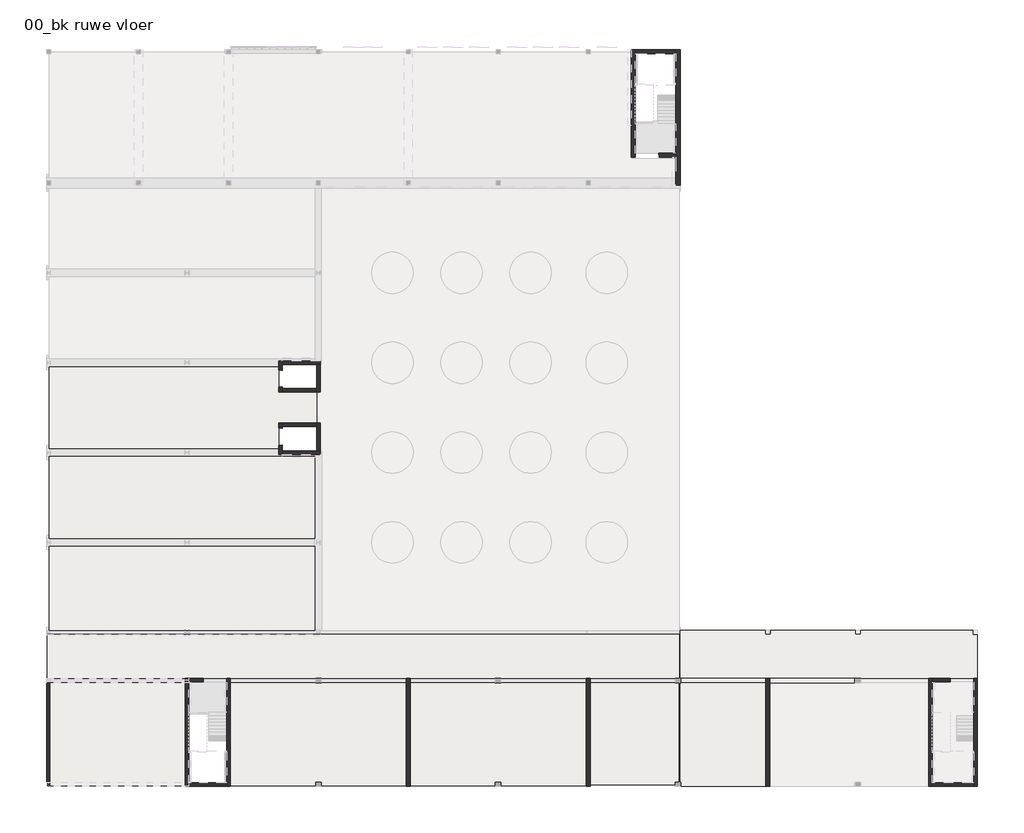
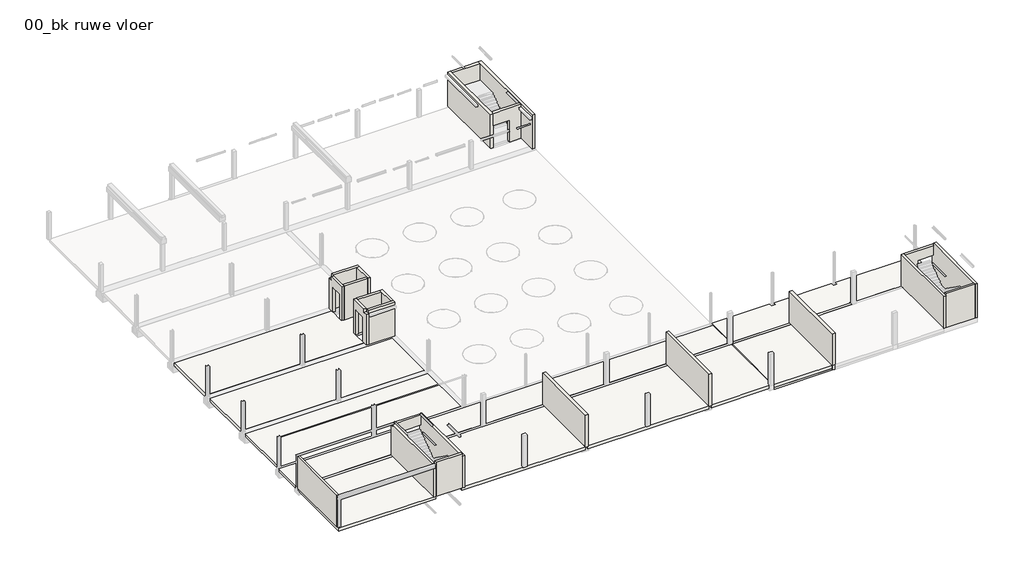
# One storey, part 1 of 6: 24 walls, 18 slabs.
"""IFC4 building model written with IfcOpenShell, lengths in millimetres."""

from ifc_helpers import new_model, si_unit, frame, origin, place, context, project, spatial, polyline, outline, extrude, faceted_brep, element, save

model = new_model("IFC4")

# Units and contexts
model_context = context("Model", 3, world=origin())
ifc_project = project(units=[si_unit("LENGTHUNIT", "METRE", prefix="MILLI")], contexts=[model_context])

# Site, building, storey
site = spatial("IfcSite", under=ifc_project)
building = spatial("IfcBuilding", under=site)
storey = spatial("IfcBuildingStorey", under=building, Name="00_bk ruwe vloer", Elevation=-70.0)

# Slabs
placement = place(None, origin())
element("IfcSlab", 1, ObjectType="NLRS_23_FL_isolatieplaatvloer 320_gen_rsf", at=placement, inside=storey, context=model_context, shape_type="Brep", body=[
    faceted_brep([(52150.0, 7650.0, -390.0), (52150.0, 11150.0, -390.0), (58300.0, 11150.0, -390.0), (58300.0, 10850.0, -390.0), (58700.0, 10850.0, -390.0), (58700.0, 11150.0, -390.0), (64800.0, 11150.0, -390.0), (64800.0, 10850.0, -390.0), (65200.0, 10850.0, -390.0), (65200.0, 11150.0, -390.0), (73300.0, 11150.0, -390.0), (73300.0, 10800.0, -390.0), (73650.0, 10800.0, -390.0), (73650.0, 7650.0, -390.0), (65250.0, 7650.0, -390.0), (65250.0, 7700.0, -390.0), (64750.0, 7700.0, -390.0), (64750.0, 7650.0, -390.0), (52150.0, 7650.0, -70.0), (64750.0, 7650.0, -70.0), (64750.0, 7700.0, -70.0), (65250.0, 7700.0, -70.0), (65250.0, 7650.0, -70.0), (73650.0, 7650.0, -70.0), (73650.0, 10800.0, -70.0), (73300.0, 10800.0, -70.0), (73300.0, 11150.0, -70.0), (65200.0, 11150.0, -70.0), (65200.0, 10850.0, -70.0), (64800.0, 10850.0, -70.0), (64800.0, 11150.0, -70.0), (58700.0, 11150.0, -70.0), (58700.0, 10850.0, -70.0), (58300.0, 10850.0, -70.0), (58300.0, 11150.0, -70.0), (52150.0, 11150.0, -70.0), (52150.0, 10850.0, -70.0)], [[[0, 1, 2, 3, 4, 5, 6, 7, 8, 9, 10, 11, 12, 13, 14, 15, 16, 17]], [[18, 19, 20, 21, 22, 23, 24, 25, 26, 27, 28, 29, 30, 31, 32, 33, 34, 35, 36]], [[1, 0, 18, 36, 35]], [[10, 9, 27, 26]], [[13, 12, 24, 23]], [[0, 17, 19, 18]], [[14, 13, 23, 22]], [[15, 14, 22, 21]], [[16, 15, 21, 20]], [[17, 16, 20, 19]], [[2, 1, 35, 34]], [[3, 2, 34, 33]], [[4, 3, 33, 32]], [[5, 4, 32, 31]], [[6, 5, 31, 30]], [[7, 6, 30, 29]], [[8, 7, 29, 28]], [[9, 8, 28, 27]], [[11, 10, 26, 25]], [[12, 11, 25, 24]]]),
])
element("IfcSlab", 2, ObjectType="NLRS_23_FL_breedplaat 320_gen_rsf", at=placement, inside=storey, context=model_context, shape_type="Brep", body=[
    faceted_brep([(6410.0, 7350.0, -390.0), (16375.0, 7350.0, -390.0), (16625.0, 7350.0, -390.0), (16625.0, 150.0, -390.0), (16625.0, -90.0, -390.0), (6650.0, -90.0, -390.0), (6410.0, -90.0, -390.0), (6410.0, 7150.0, -390.0), (16400.0, 125.0, -390.0), (16400.0, 7175.0, -390.0), (6625.0, 7175.0, -390.0), (6625.0, 125.0, -390.0), (16625.0, 7350.0, -70.0), (6410.0, 7350.0, -70.0), (6410.0, -90.0, -70.0), (6650.0, -90.0, -70.0), (16625.0, -90.0, -70.0), (16625.0, 150.0, -70.0), (6625.0, 7175.0, -330.0), (16400.0, 7175.0, -330.0), (16400.0, 125.0, -330.0), (6625.0, 125.0, -330.0)], [[[0, 1, 2, 3, 4, 5, 6, 7], [8, 9, 10, 11]], [[12, 13, 14, 15, 16, 17]], [[2, 1, 0, 13, 12]], [[4, 3, 2, 12, 17, 16]], [[6, 5, 4, 16, 15, 14]], [[0, 7, 6, 14, 13]], [[18, 19, 20, 21]], [[20, 19, 9, 8]], [[21, 20, 8, 11]], [[18, 21, 11, 10]], [[19, 18, 10, 9]]]),
])
element("IfcSlab", 3, ObjectType="NLRS_23_FL_breedplaat 320_gen_rsf", at=placement, inside=storey, context=model_context, shape_type="Brep", body=[
    faceted_brep([(52090.0, 10850.0, -390.0), (52090.0, 10650.0, -390.0), (52090.0, 7850.0, -390.0), (52090.0, 7650.0, -390.0), (19375.0, 7650.0, -390.0), (16625.0, 7650.0, -390.0), (16375.0, 7650.0, -390.0), (6410.0, 7650.0, -390.0), (6410.0, 7850.0, -390.0), (6410.0, 10650.0, -390.0), (6410.0, 10850.0, -390.0), (51875.0, 7825.0, -390.0), (51875.0, 10675.0, -390.0), (6625.0, 10675.0, -390.0), (6625.0, 7825.0, -390.0), (52090.0, 7650.0, -70.0), (52090.0, 10850.0, -70.0), (6410.0, 10850.0, -70.0), (6410.0, 7650.0, -70.0), (16625.0, 7650.0, -70.0), (19375.0, 7650.0, -70.0), (6625.0, 10675.0, -330.0), (51875.0, 10675.0, -330.0), (51875.0, 7825.0, -330.0), (6625.0, 7825.0, -330.0)], [[[0, 1, 2, 3, 4, 5, 6, 7, 8, 9, 10], [11, 12, 13, 14]], [[15, 16, 17, 18, 19, 20]], [[3, 2, 1, 0, 16, 15]], [[7, 6, 5, 4, 3, 15, 20, 19, 18]], [[10, 9, 8, 7, 18, 17]], [[0, 10, 17, 16]], [[21, 22, 23, 24]], [[23, 22, 12, 11]], [[24, 23, 11, 14]], [[21, 24, 14, 13]], [[22, 21, 13, 12]]]),
])
element("IfcSlab", 4, ObjectType="NLRS_23_FL_isolatieplaatvloer 320_gen_rsf", at=placement, inside=storey, context=model_context, shape_type="Brep", body=[
    faceted_brep([(25750.0, 17200.0, -390.0), (25750.0, 11350.0, -390.0), (25750.0, 11150.0, -390.0), (6550.0, 11150.0, -390.0), (6550.0, 11350.0, -390.0), (6550.0, 17000.0, -390.0), (6550.0, 17200.0, -390.0), (25500.0, 17200.0, -390.0), (25550.0, 17200.0, -390.0), (25700.0, 17200.0, -390.0), (25750.0, 17200.0, -70.0), (25700.0, 17200.0, -70.0), (6550.0, 17200.0, -70.0), (6550.0, 11150.0, -70.0), (25750.0, 11150.0, -70.0)], [[[0, 1, 2, 3, 4, 5, 6, 7, 8, 9]], [[10, 11, 12, 13, 14]], [[2, 1, 0, 10, 14]], [[3, 2, 14, 13]], [[6, 5, 4, 3, 13, 12]], [[0, 9, 8, 7, 6, 12, 11, 10]]]),
])
element("IfcSlab", 5, ObjectType="NLRS_23_FL_isolatieplaatvloer 320_gen_rsf", at=placement, inside=storey, context=model_context, shape_type="Brep", body=[
    faceted_brep([(25750.0, 23700.0, -390.0), (25750.0, 17800.0, -390.0), (25700.0, 17800.0, -390.0), (25550.0, 17800.0, -390.0), (25500.0, 17800.0, -390.0), (6550.0, 17800.0, -390.0), (6550.0, 18000.0, -390.0), (6550.0, 23500.0, -390.0), (6550.0, 23700.0, -390.0), (25500.0, 23700.0, -390.0), (25550.0, 23700.0, -390.0), (25700.0, 23700.0, -390.0), (25750.0, 23700.0, -70.0), (25700.0, 23700.0, -70.0), (6550.0, 23700.0, -70.0), (6550.0, 17800.0, -70.0), (25700.0, 17800.0, -70.0), (25750.0, 17800.0, -70.0)], [[[0, 1, 2, 3, 4, 5, 6, 7, 8, 9, 10, 11]], [[12, 13, 14, 15, 16, 17]], [[1, 0, 12, 17]], [[5, 4, 3, 2, 1, 17, 16, 15]], [[8, 7, 6, 5, 15, 14]], [[0, 11, 10, 9, 8, 14, 13, 12]]]),
])
element("IfcSlab", 6, ObjectType="NLRS_23_FL_isolatieplaatvloer 320_gen_rsf", at=placement, inside=storey, context=model_context, shape_type="Brep", body=[
    faceted_brep([(23125.0, 30200.0, -390.0), (23125.0, 30000.0, -390.0), (23125.0, 28475.0, -390.0), (23375.0, 28475.0, -390.0), (25875.0, 28475.0, -390.0), (25875.0, 28375.0, -390.0), (25875.0, 26125.0, -390.0), (25875.0, 26025.0, -390.0), (23375.0, 26025.0, -390.0), (23125.0, 26025.0, -390.0), (23125.0, 24500.0, -390.0), (23125.0, 24300.0, -390.0), (6550.0, 24300.0, -390.0), (6550.0, 24500.0, -390.0), (6550.0, 30000.0, -390.0), (6550.0, 30200.0, -390.0), (23125.0, 30200.0, -70.0), (6550.0, 30200.0, -70.0), (6550.0, 24300.0, -70.0), (23125.0, 24300.0, -70.0), (23125.0, 26025.0, -70.0), (23375.0, 26025.0, -70.0), (25875.0, 26025.0, -70.0), (25875.0, 28475.0, -70.0), (23375.0, 28475.0, -70.0), (23125.0, 28475.0, -70.0)], [[[0, 1, 2, 3, 4, 5, 6, 7, 8, 9, 10, 11, 12, 13, 14, 15]], [[16, 17, 18, 19, 20, 21, 22, 23, 24, 25]], [[2, 1, 0, 16, 25]], [[12, 11, 19, 18]], [[15, 14, 13, 12, 18, 17]], [[0, 15, 17, 16]], [[4, 3, 2, 25, 24, 23]], [[7, 6, 5, 4, 23, 22]], [[9, 8, 7, 22, 21, 20]], [[11, 10, 9, 20, 19]]]),
])
element("IfcSlab", 7, ObjectType="NLRS_23_FL_breedplaat 320_gen_rsf", at=placement, inside=storey, context=model_context, shape_type="Brep", body=[
    faceted_brep([(32350.0, 7350.0, -390.0), (32350.0, 150.0, -390.0), (32350.0, -90.0, -390.0), (19375.0, -90.0, -390.0), (19375.0, 150.0, -390.0), (19375.0, 7350.0, -390.0), (32175.0, 125.0, -390.0), (32175.0, 7175.0, -390.0), (19600.0, 7175.0, -390.0), (19600.0, 125.0, -390.0), (32350.0, -90.0, -70.0), (32350.0, 150.0, -70.0), (32350.0, 7350.0, -70.0), (19375.0, 7350.0, -70.0), (19375.0, 150.0, -70.0), (19375.0, -90.0, -70.0), (19600.0, 7175.0, -330.0), (32175.0, 7175.0, -330.0), (32175.0, 125.0, -330.0), (19600.0, 125.0, -330.0)], [[[0, 1, 2, 3, 4, 5], [6, 7, 8, 9]], [[10, 11, 12, 13, 14, 15]], [[2, 1, 0, 12, 11, 10]], [[3, 2, 10, 15]], [[5, 4, 3, 15, 14, 13]], [[0, 5, 13, 12]], [[16, 17, 18, 19]], [[18, 17, 7, 6]], [[19, 18, 6, 9]], [[16, 19, 9, 8]], [[17, 16, 8, 7]]]),
])
element("IfcSlab", 8, ObjectType="NLRS_23_FL_breedplaat 320_gen_rsf", at=placement, inside=storey, context=model_context, shape_type="Brep", body=[
    faceted_brep([(45350.0, 7350.0, -390.0), (45350.0, 7150.0, -390.0), (45350.0, 150.0, -390.0), (45350.0, -90.0, -390.0), (32650.0, -90.0, -390.0), (32650.0, 150.0, -390.0), (32650.0, 7150.0, -390.0), (32650.0, 7350.0, -390.0), (45175.0, 125.0, -390.0), (45175.0, 7175.0, -390.0), (32825.0, 7175.0, -390.0), (32825.0, 125.0, -390.0), (45350.0, -90.0, -70.0), (45350.0, 150.0, -70.0), (45350.0, 7350.0, -70.0), (32650.0, 7350.0, -70.0), (32650.0, 150.0, -70.0), (32650.0, -90.0, -70.0), (32825.0, 7175.0, -330.0), (45175.0, 7175.0, -330.0), (45175.0, 125.0, -330.0), (32825.0, 125.0, -330.0)], [[[0, 1, 2, 3, 4, 5, 6, 7], [8, 9, 10, 11]], [[12, 13, 14, 15, 16, 17]], [[3, 2, 1, 0, 14, 13, 12]], [[4, 3, 12, 17]], [[7, 6, 5, 4, 17, 16, 15]], [[0, 7, 15, 14]], [[18, 19, 20, 21]], [[20, 19, 9, 8]], [[21, 20, 8, 11]], [[18, 21, 11, 10]], [[19, 18, 10, 9]]]),
])
element("IfcSlab", 9, ObjectType="NLRS_23_FL_breedplaat 320_gen_rsf", at=placement, inside=storey, context=model_context, shape_type="Brep", body=[
    faceted_brep([(52050.0, 7350.0, -390.0), (52050.0, 7150.0, -390.0), (52050.0, 150.0, -390.0), (52050.0, -50.0, -390.0), (51750.0, -50.0, -390.0), (45650.0, -50.0, -390.0), (45650.0, 150.0, -390.0), (45650.0, 7150.0, -390.0), (45650.0, 7350.0, -390.0), (51875.0, 125.0, -390.0), (51875.0, 7175.0, -390.0), (45825.0, 7175.0, -390.0), (45825.0, 125.0, -390.0), (52050.0, -50.0, -70.0), (52050.0, 150.0, -70.0), (52050.0, 7350.0, -70.0), (45650.0, 7350.0, -70.0), (45650.0, 150.0, -70.0), (45650.0, -50.0, -70.0), (51750.0, -50.0, -70.0), (45825.0, 7175.0, -330.0), (51875.0, 7175.0, -330.0), (51875.0, 125.0, -330.0), (45825.0, 125.0, -330.0)], [[[0, 1, 2, 3, 4, 5, 6, 7, 8], [9, 10, 11, 12]], [[13, 14, 15, 16, 17, 18, 19]], [[3, 2, 1, 0, 15, 14, 13]], [[5, 4, 3, 13, 19, 18]], [[8, 7, 6, 5, 18, 17, 16]], [[0, 8, 16, 15]], [[20, 21, 22, 23]], [[22, 21, 10, 9]], [[23, 22, 9, 12]], [[20, 23, 12, 11]], [[21, 20, 11, 10]]]),
])
element("IfcSlab", 10, ObjectType="NLRS_23_FL_isolatieplaatvloer 320_gen_rsf", at=placement, inside=storey, context=model_context, shape_type="SweptSolid", body=[
    extrude(outline(polyline([(58350.0, 7350.0), (58350.0, -150.0), (52250.0, -150.0), (52250.0, 150.0), (52150.0, 150.0), (52150.0, 7350.0), (58350.0, 7350.0)])), frame((0.0, 0.0, -390.0), z_axis=(0.0, 0.0, 1.0), x_axis=(1.0, 0.0, 0.0)), (0.0, 0.0, 1.0), 320.0),
])
element("IfcSlab", 11, ObjectType="NLRS_23_FL_beton ihwg vloeraanstort 520_gen_rsf", at=placement, inside=storey, context=model_context, shape_type="Brep", body=[
    faceted_brep([(64750.0, 7650.0, -590.0), (64750.0, 7350.0, -590.0), (58650.0, 7350.0, -590.0), (58650.0, -150.0, -590.0), (58350.0, -150.0, -590.0), (58350.0, 7350.0, -590.0), (52150.0, 7350.0, -590.0), (52150.0, 7650.0, -590.0), (64750.0, 7650.0, -70.0), (52200.0, 7650.0, -70.0), (52150.0, 7650.0, -70.0), (52150.0, 7350.0, -70.0), (52200.0, 7350.0, -70.0), (58350.0, 7350.0, -70.0), (58350.0, -150.0, -70.0), (58650.0, -150.0, -70.0), (58650.0, 7350.0, -70.0), (64750.0, 7350.0, -70.0), (52150.0, 7350.0, -390.0), (52150.0, 7650.0, -390.0)], [[[0, 1, 2, 3, 4, 5, 6, 7]], [[8, 9, 10, 11, 12, 13, 14, 15, 16, 17]], [[1, 0, 8, 17]], [[2, 1, 17, 16]], [[3, 2, 16, 15]], [[4, 3, 15, 14]], [[5, 4, 14, 13]], [[6, 5, 13, 12, 11, 18]], [[7, 6, 18, 11, 10, 19]], [[0, 7, 19, 10, 9, 8]]]),
])
element("IfcSlab", 12, ObjectType="NLRS_23_FL_isolatie isolatieplaatvloer 200_gen_rsf", at=placement, inside=storey, context=model_context, shape_type="Brep", body=[
    faceted_brep([(52150.0, 7650.0, -590.0), (52150.0, 7800.0, -590.0), (52150.0, 10750.0, -590.0), (52150.0, 11150.0, -590.0), (58300.0, 11150.0, -590.0), (58300.0, 10850.0, -590.0), (58700.0, 10850.0, -590.0), (58700.0, 11150.0, -590.0), (64800.0, 11150.0, -590.0), (64800.0, 10850.0, -590.0), (65200.0, 10850.0, -590.0), (65200.0, 11150.0, -590.0), (73300.0, 11150.0, -590.0), (73300.0, 10800.0, -590.0), (73650.0, 10800.0, -590.0), (73650.0, 7650.0, -590.0), (65250.0, 7650.0, -590.0), (65250.0, 7700.0, -590.0), (64750.0, 7700.0, -590.0), (64750.0, 7650.0, -590.0), (52150.0, 7650.0, -390.0), (64750.0, 7650.0, -390.0), (64750.0, 7700.0, -390.0), (65250.0, 7700.0, -390.0), (65250.0, 7650.0, -390.0), (73650.0, 7650.0, -390.0), (73650.0, 10800.0, -390.0), (73300.0, 10800.0, -390.0), (73300.0, 11150.0, -390.0), (65200.0, 11150.0, -390.0), (65200.0, 10850.0, -390.0), (64800.0, 10850.0, -390.0), (64800.0, 11150.0, -390.0), (58700.0, 11150.0, -390.0), (58700.0, 10850.0, -390.0), (58300.0, 10850.0, -390.0), (58300.0, 11150.0, -390.0), (52150.0, 11150.0, -390.0), (52150.0, 10850.0, -390.0), (52150.0, 10650.0, -390.0), (52150.0, 7850.0, -390.0)], [[[0, 1, 2, 3, 4, 5, 6, 7, 8, 9, 10, 11, 12, 13, 14, 15, 16, 17, 18, 19]], [[20, 21, 22, 23, 24, 25, 26, 27, 28, 29, 30, 31, 32, 33, 34, 35, 36, 37, 38, 39, 40]], [[3, 2, 1, 0, 20, 40, 39, 38, 37]], [[12, 11, 29, 28]], [[15, 14, 26, 25]], [[0, 19, 21, 20]], [[16, 15, 25, 24]], [[17, 16, 24, 23]], [[18, 17, 23, 22]], [[19, 18, 22, 21]], [[4, 3, 37, 36]], [[5, 4, 36, 35]], [[6, 5, 35, 34]], [[7, 6, 34, 33]], [[8, 7, 33, 32]], [[9, 8, 32, 31]], [[10, 9, 31, 30]], [[11, 10, 30, 29]], [[13, 12, 28, 27]], [[14, 13, 27, 26]]]),
])
element("IfcSlab", 13, ObjectType="NLRS_23_FL_isolatie isolatieplaatvloer 200_gen_rsf", at=placement, inside=storey, context=model_context, shape_type="Brep", body=[
    faceted_brep([(58350.0, 7350.0, -590.0), (58350.0, -150.0, -590.0), (52250.0, -150.0, -590.0), (52250.0, 150.0, -590.0), (52150.0, 150.0, -590.0), (52150.0, 250.0, -590.0), (52150.0, 7200.0, -590.0), (52150.0, 7350.0, -590.0), (58350.0, 7350.0, -390.0), (52150.0, 7350.0, -390.0), (52150.0, 7150.0, -390.0), (52150.0, 150.0, -390.0), (52250.0, 150.0, -390.0), (52250.0, -150.0, -390.0), (58350.0, -150.0, -390.0)], [[[0, 1, 2, 3, 4, 5, 6, 7]], [[8, 9, 10, 11, 12, 13, 14]], [[1, 0, 8, 14]], [[2, 1, 14, 13]], [[7, 6, 5, 4, 11, 10, 9]], [[0, 7, 9, 8]], [[3, 2, 13, 12]], [[4, 3, 12, 11]]]),
])
element("IfcSlab", 14, ObjectType="NLRS_23_FL_breedplaat schil 60_gen_rsf", at=placement, inside=storey, context=model_context, shape_type="SweptSolid", body=[
    extrude(outline(polyline([(16400.0, 7175.0), (16400.0, 125.0), (6625.0, 125.0), (6625.0, 7175.0), (16400.0, 7175.0)])), frame((0.0, 0.0, -390.0), z_axis=(0.0, 0.0, 1.0), x_axis=(1.0, 0.0, 0.0)), (0.0, 0.0, 1.0), 60.0),
])
element("IfcSlab", 15, ObjectType="NLRS_23_FL_breedplaat schil 60_gen_rsf", at=placement, inside=storey, context=model_context, shape_type="SweptSolid", body=[
    extrude(outline(polyline([(32175.0, 7175.0), (32175.0, 125.0), (19600.0, 125.0), (19600.0, 7175.0), (32175.0, 7175.0)])), frame((0.0, 0.0, -390.0), z_axis=(0.0, 0.0, 1.0), x_axis=(1.0, 0.0, 0.0)), (0.0, 0.0, 1.0), 60.0),
])
element("IfcSlab", 16, ObjectType="NLRS_23_FL_breedplaat schil 60_gen_rsf", at=placement, inside=storey, context=model_context, shape_type="SweptSolid", body=[
    extrude(outline(polyline([(45175.0, 7175.0), (45175.0, 125.0), (32825.0, 125.0), (32825.0, 7175.0), (45175.0, 7175.0)])), frame((0.0, 0.0, -390.0), z_axis=(0.0, 0.0, 1.0), x_axis=(1.0, 0.0, 0.0)), (0.0, 0.0, 1.0), 60.0),
])
element("IfcSlab", 17, ObjectType="NLRS_23_FL_breedplaat schil 60_gen_rsf", at=placement, inside=storey, context=model_context, shape_type="SweptSolid", body=[
    extrude(outline(polyline([(51875.0, 7175.0), (51875.0, 125.0), (45825.0, 125.0), (45825.0, 7175.0), (51875.0, 7175.0)])), frame((0.0, 0.0, -390.0), z_axis=(0.0, 0.0, 1.0), x_axis=(1.0, 0.0, 0.0)), (0.0, 0.0, 1.0), 60.0),
])
element("IfcSlab", 18, ObjectType="NLRS_23_FL_breedplaat schil 60_gen_rsf", at=placement, inside=storey, context=model_context, shape_type="SweptSolid", body=[
    extrude(outline(polyline([(51875.0, 10675.0), (51875.0, 7825.0), (6625.0, 7825.0), (6625.0, 10675.0), (51875.0, 10675.0)])), frame((0.0, 0.0, -390.0), z_axis=(0.0, 0.0, 1.0), x_axis=(1.0, 0.0, 0.0)), (0.0, 0.0, 1.0), 60.0),
])

# Walls
element("IfcWall", 19, ObjectType="NLRS_22_WA_beton ihw 250_gen_rsf", at=placement, inside=storey, context=model_context, shape_type="Brep", body=[
    faceted_brep([(19625.0, -150.0, -70.0), (19625.0, 7650.0, -70.0), (19625.0, 7650.0, 3470.0), (19625.0, -150.0, 3470.0), (19375.0, -150.0, -70.0), (19375.0, -150.0, 3470.0), (19375.0, 7400.0, 3470.0), (19375.0, 7650.0, 3470.0), (19375.0, 7650.0, 2370.0), (19375.0, 7650.0, -70.0), (19375.0, 7350.0, -70.0), (19375.0, 100.0, -70.0), (19375.0, -90.0, -70.0)], [[[0, 1, 2, 3]], [[4, 5, 6, 7, 8, 9, 10, 11, 12]], [[1, 0, 4, 12, 11, 10, 9]], [[2, 1, 9, 8, 7]], [[3, 2, 7, 6, 5]], [[0, 3, 5, 4]]]),
])
element("IfcWall", 20, ObjectType="NLRS_22_WA_beton ihw 250_gen_rsf", at=placement, inside=storey, context=model_context, shape_type="Brep", body=[
    faceted_brep([(16625.0, -150.0, -70.0), (16625.0, -90.0, -70.0), (16625.0, 100.0, -70.0), (16625.0, 7350.0, -70.0), (16625.0, 7400.0, -70.0), (16625.0, 7650.0, -70.0), (16625.0, 7650.0, 3320.0), (16625.0, 7330.0, 3320.0), (16625.0, 7330.0, 3470.0), (16625.0, 170.0, 3470.0), (16625.0, 170.0, 3090.0), (16625.0, -150.0, 3090.0), (16375.0, -150.0, -70.0), (16375.0, -150.0, 3090.0), (16375.0, 170.0, 3090.0), (16375.0, 170.0, 3470.0), (16375.0, 7330.0, 3470.0), (16375.0, 7330.0, 3320.0), (16375.0, 7650.0, 3320.0), (16375.0, 7650.0, -70.0)], [[[0, 1, 2, 3, 4, 5, 6, 7, 8, 9, 10, 11]], [[12, 13, 14, 15, 16, 17, 18, 19]], [[5, 4, 3, 2, 1, 0, 12, 19]], [[6, 5, 19, 18]], [[9, 8, 16, 15]], [[0, 11, 13, 12]], [[10, 9, 15, 14]], [[11, 10, 14, 13]], [[7, 6, 18, 17]], [[8, 7, 17, 16]]]),
])
element("IfcWall", 21, ObjectType="NLRS_22_WA_kalkzandsteen CS20 300_gen_rsf", at=placement, inside=storey, context=model_context, shape_type="SweptSolid", body=[
    extrude(outline(polyline([(32650.0, 7650.0), (32650.0, -150.0), (32350.0, -150.0), (32350.0, 7650.0), (32650.0, 7650.0)])), frame((0.0, 0.0, -70.0), z_axis=(0.0, 0.0, 1.0), x_axis=(1.0, 0.0, 0.0)), (0.0, 0.0, 1.0), 3540.0),
])
element("IfcWall", 22, ObjectType="NLRS_22_WA_kalkzandsteen CS20 300_gen_rsf", at=placement, inside=storey, context=model_context, shape_type="SweptSolid", body=[
    extrude(outline(polyline([(45650.0, 7650.0), (45650.0, -150.0), (45350.0, -150.0), (45350.0, 7650.0), (45650.0, 7650.0)])), frame((0.0, 0.0, -70.0), z_axis=(0.0, 0.0, 1.0), x_axis=(1.0, 0.0, 0.0)), (0.0, 0.0, 1.0), 3540.0),
])
element("IfcWall", 23, ObjectType="NLRS_22_WA_kalkzandsteen CS20 300_gen_rsf", at=placement, inside=storey, context=model_context, shape_type="SweptSolid", body=[
    extrude(outline(polyline([(58650.0, 7650.0), (58650.0, -150.0), (58350.0, -150.0), (58350.0, 7650.0), (58650.0, 7650.0)])), frame((0.0, 0.0, -70.0), z_axis=(0.0, 0.0, 1.0), x_axis=(1.0, 0.0, 0.0)), (0.0, 0.0, 1.0), 3540.0),
])
element("IfcWall", 24, ObjectType="NLRS_21_WA_beton ihw 250_gen_rsf", at=placement, inside=storey, context=model_context, shape_type="Brep", body=[
    faceted_brep([(73650.0, -150.0, -70.0), (73650.0, 7650.0, -70.0), (73650.0, 7650.0, 3470.0), (73650.0, 7400.0, 3470.0), (73650.0, 7400.0, 3730.0), (73650.0, -150.0, 3730.0), (73400.0, -150.0, -70.0), (73400.0, -150.0, 3730.0), (73400.0, 100.0, 3730.0), (73400.0, 7400.0, 3730.0), (73400.0, 7400.0, 3470.0), (73400.0, 7650.0, 3470.0), (73400.0, 7650.0, 2370.0), (73400.0, 7650.0, -70.0), (73400.0, 7400.0, -70.0), (73400.0, 100.0, -70.0)], [[[0, 1, 2, 3, 4, 5]], [[6, 7, 8, 9, 10, 11, 12, 13, 14, 15]], [[1, 0, 6, 15, 14, 13]], [[2, 1, 13, 12, 11]], [[5, 4, 9, 8, 7]], [[0, 5, 7, 6]], [[3, 2, 11, 10]], [[4, 3, 10, 9]]]),
])
element("IfcWall", 25, ObjectType="NLRS_21_WA_kalkzandsteen CS12 214_gen_rsf", at=placement, inside=storey, context=model_context, shape_type="SweptSolid", body=[
    extrude(outline(polyline([(6564.0, 7330.0), (6564.0, 170.0), (6350.0, 170.0), (6350.0, 7330.0), (6564.0, 7330.0)])), frame((0.0, 0.0, -70.0), z_axis=(0.0, 0.0, 1.0), x_axis=(1.0, 0.0, 0.0)), (0.0, 0.0, 1.0), 3540.0),
])
element("IfcWall", 26, ObjectType="NLRS_21_WA_beton ihw 250_gen_rsf", at=placement, inside=storey, context=model_context, shape_type="Brep", body=[
    faceted_brep([(16625.0, -150.0, -70.0), (19375.0, -150.0, -70.0), (19375.0, -150.0, 3470.0), (19375.0, -150.0, 3730.0), (16625.0, -150.0, 3730.0), (16625.0, -150.0, 3470.0), (16625.0, -150.0, 3090.0), (19375.0, 100.0, -70.0), (16625.0, 100.0, -70.0), (16625.0, 100.0, 3730.0), (19375.0, 100.0, 3730.0), (19375.0, 100.0, 3470.0)], [[[0, 1, 2, 3, 4, 5, 6]], [[7, 8, 9, 10, 11]], [[1, 0, 8, 7]], [[1, 7, 11, 10, 3, 2]], [[4, 3, 10, 9]], [[0, 6, 5, 4, 9, 8]]]),
])
element("IfcWall", 27, ObjectType="NLRS_22_WA_beton ihw 250_gen_rsf", at=placement, inside=storey, context=model_context, shape_type="Brep", body=[
    faceted_brep([(19375.0, 7400.0, 3470.0), (16625.0, 7400.0, 3470.0), (16625.0, 7400.0, -70.0), (17675.0, 7400.0, -70.0), (17675.0, 7400.0, 2370.0), (19375.0, 7400.0, 2370.0), (16625.0, 7650.0, 3470.0), (19375.0, 7650.0, 3470.0), (19375.0, 7650.0, 2370.0), (17675.0, 7650.0, 2370.0), (17675.0, 7650.0, -70.0), (16625.0, 7650.0, -70.0), (16625.0, 7650.0, 3320.0)], [[[0, 1, 2, 3, 4, 5]], [[6, 7, 8, 9, 10, 11, 12]], [[2, 11, 10, 3]], [[7, 0, 5, 8]], [[1, 0, 7, 6]], [[2, 1, 6, 12, 11]], [[9, 4, 3, 10]], [[4, 9, 8, 5]]]),
])
element("IfcWall", 28, ObjectType="NLRS_22_WA_beton ihw 250_gen_rsf", at=placement, inside=storey, context=model_context, shape_type="Brep", body=[
    faceted_brep([(70375.0, -150.0, -70.0), (70375.0, 100.0, -70.0), (70375.0, 7400.0, -70.0), (70375.0, 7650.0, -70.0), (70375.0, 7650.0, 3470.0), (70375.0, 7400.0, 3470.0), (70375.0, -150.0, 3470.0), (70125.0, -150.0, -70.0), (70125.0, -150.0, 3470.0), (70125.0, 7650.0, 3470.0), (70125.0, 7650.0, -70.0), (70125.0, 7350.0, -70.0)], [[[0, 1, 2, 3, 4, 5, 6]], [[7, 8, 9, 10, 11]], [[3, 2, 1, 0, 7, 11, 10]], [[4, 3, 10, 9]], [[6, 5, 4, 9, 8]], [[0, 6, 8, 7]]]),
])
element("IfcWall", 29, ObjectType="NLRS_21_WA_beton ihw 250_gen_rsf", at=placement, inside=storey, context=model_context, shape_type="Brep", body=[
    faceted_brep([(70375.0, -150.0, -70.0), (73400.0, -150.0, -70.0), (73400.0, -150.0, 3730.0), (70375.0, -150.0, 3730.0), (70375.0, -150.0, 3470.0), (70375.0, 100.0, -70.0), (70375.0, 100.0, 3730.0), (73400.0, 100.0, 3730.0), (73400.0, 100.0, -70.0)], [[[0, 1, 2, 3, 4]], [[5, 6, 7, 8]], [[1, 0, 5, 8]], [[2, 1, 8, 7]], [[3, 2, 7, 6]], [[0, 4, 3, 6, 5]]]),
])
element("IfcWall", 30, ObjectType="NLRS_22_WA_beton ihw 250_gen_rsf", at=placement, inside=storey, context=model_context, shape_type="SweptSolid", body=[
    extrude(outline(polyline([(3470.0, 73400.0), (3470.0, 70375.0), (-70.0, 70375.0), (-70.0, 71700.0), (2370.0, 71700.0), (2370.0, 73400.0), (3470.0, 73400.0)])), frame((0.0, 7400.0, 0.0), z_axis=(0.0, 1.0, 0.0), x_axis=(0.0, 0.0, 1.0)), (0.0, 0.0, 1.0), 250.0),
])
element("IfcWall", 31, ObjectType="NLRS_22_WA_beton prefab 300_gen_rsf", at=placement, inside=storey, context=model_context, shape_type="Brep", body=[
    faceted_brep([(48905.0, 45350.0, -50.0), (48905.0, 53150.0, -50.0), (48905.0, 53150.0, 3730.0), (48905.0, 45350.0, 3730.0), (48605.0, 45350.0, -50.0), (48605.0, 45350.0, 3730.0), (48605.0, 53150.0, 3730.0), (48605.0, 53150.0, 3470.0), (48605.0, 53150.0, 3220.0), (48605.0, 53150.0, -50.0)], [[[0, 1, 2, 3]], [[4, 5, 6, 7, 8, 9]], [[1, 0, 4, 9]], [[2, 1, 9, 8, 7, 6]], [[3, 2, 6, 5]], [[0, 3, 5, 4]]]),
])
element("IfcWall", 32, ObjectType="NLRS_21_WA_beton prefab 300_gen_rsf", at=placement, inside=storey, context=model_context, shape_type="Brep", body=[
    faceted_brep([(52150.0, 43350.0, -50.0), (52150.0, 53150.0, -50.0), (52150.0, 53150.0, 3730.0), (52150.0, 43350.0, 3730.0), (51850.0, 43350.0, -50.0), (51850.0, 43350.0, 3220.0), (51850.0, 43350.0, 3470.0), (51850.0, 43350.0, 3730.0), (51850.0, 53150.0, 3730.0), (51850.0, 53150.0, -50.0)], [[[0, 1, 2, 3]], [[4, 5, 6, 7, 8, 9]], [[1, 0, 4, 9]], [[2, 1, 9, 8]], [[3, 2, 8, 7]], [[0, 3, 7, 6, 5, 4]]]),
])
element("IfcWall", 33, ObjectType="NLRS_21_WA_beton prefab 300_gen_rsf", at=placement, inside=storey, context=model_context, shape_type="SweptSolid", body=[
    extrude(outline(polyline([(48925.0, 53150.0), (51830.0, 53150.0), (51830.0, 52850.0), (48925.0, 52850.0), (48925.0, 53150.0)])), frame((0.0, 0.0, -50.0), z_axis=(0.0, 0.0, 1.0), x_axis=(1.0, 0.0, 0.0)), (0.0, 0.0, 1.0), 3780.0),
])
element("IfcWall", 34, ObjectType="NLRS_22_WA_beton prefab 300_gen_rsf", at=placement, inside=storey, context=model_context, shape_type="Brep", body=[
    faceted_brep([(48925.0, 45650.0, 3730.0), (51830.0, 45650.0, 3730.0), (51830.0, 45650.0, -50.0), (50625.0, 45650.0, -50.0), (50625.0, 45650.0, 2370.0), (48925.0, 45650.0, 2370.0), (51830.0, 45350.0, 3730.0), (48925.0, 45350.0, 3730.0), (48925.0, 45350.0, 2400.0), (50655.0, 45350.0, 2400.0), (50655.0, 45350.0, -50.0), (51830.0, 45350.0, -50.0)], [[[0, 1, 2, 3, 4, 5]], [[6, 7, 8, 9, 10, 11]], [[2, 11, 10, 3]], [[7, 0, 5, 8]], [[1, 0, 7, 6]], [[2, 1, 6, 11]], [[9, 4, 3, 10]], [[4, 9, 8, 5]]]),
])
element("IfcWall", 35, ObjectType="NLRS_22_WA_beton prefab 250_gen_rsf", at=placement, inside=storey, context=model_context, shape_type="Brep", body=[
    faceted_brep([(26125.0, 30625.0, -40.0), (23395.0, 30625.0, -40.0), (23395.0, 30625.0, 3150.0), (23395.0, 30625.0, 3400.0), (23395.0, 30625.0, 3730.0), (26125.0, 30625.0, 3730.0), (26125.0, 30625.0, 3400.0), (26125.0, 30625.0, 3150.0), (26125.0, 30375.0, -40.0), (26125.0, 30375.0, 3730.0), (23395.0, 30375.0, 3730.0), (23395.0, 30375.0, -40.0)], [[[0, 1, 2, 3, 4, 5, 6, 7]], [[8, 9, 10, 11]], [[1, 0, 8, 11]], [[4, 3, 2, 1, 11, 10]], [[5, 4, 10, 9]], [[0, 7, 6, 5, 9, 8]]]),
])
element("IfcWall", 36, ObjectType="NLRS_22_WA_beton prefab 250_gen_rsf", at=placement, inside=storey, context=model_context, shape_type="Brep", body=[
    faceted_brep([(23125.0, 28375.0, -40.0), (23125.0, 28375.0, 3730.0), (23125.0, 30231.5, 3730.0), (23125.0, 30231.5, 3355.0), (23125.0, 30625.0, 3355.0), (23125.0, 30625.0, -40.0), (23125.0, 29973.0, -40.0), (23125.0, 29973.0, 2705.0), (23125.0, 28723.0, 2705.0), (23125.0, 28723.0, -40.0), (23375.0, 28375.0, 3730.0), (23375.0, 28375.0, -40.0), (23375.0, 28748.0, -40.0), (23375.0, 28748.0, 2680.0), (23375.0, 29948.0, 2680.0), (23375.0, 29948.0, -40.0), (23375.0, 30625.0, -40.0), (23375.0, 30625.0, 3355.0), (23375.0, 30231.5, 3355.0), (23375.0, 30231.5, 3730.0)], [[[0, 1, 2, 3, 4, 5, 6, 7, 8, 9]], [[10, 11, 12, 13, 14, 15, 16, 17, 18, 19]], [[11, 0, 9, 12]], [[5, 16, 15, 6]], [[1, 0, 11, 10]], [[2, 1, 10, 19]], [[5, 4, 17, 16]], [[3, 2, 19, 18]], [[4, 3, 18, 17]], [[14, 7, 6, 15]], [[8, 13, 12, 9]], [[7, 14, 13, 8]]]),
])
element("IfcWall", 37, ObjectType="NLRS_22_WA_beton prefab 250_gen_rsf", at=placement, inside=storey, context=model_context, shape_type="SweptSolid", body=[
    extrude(outline(polyline([(25855.0, 28375.0), (23395.0, 28375.0), (23395.0, 28625.0), (25855.0, 28625.0), (25855.0, 28375.0)])), frame((0.0, 0.0, -40.0), z_axis=(0.0, 0.0, 1.0), x_axis=(1.0, 0.0, 0.0)), (0.0, 0.0, 1.0), 3770.0),
])
element("IfcWall", 38, ObjectType="NLRS_21_WA_beton prefab 250_gen_rsf", at=placement, inside=storey, context=model_context, shape_type="SweptSolid", body=[
    extrude(outline(polyline([(26125.0, 30355.0), (26125.0, 28375.0), (25875.0, 28375.0), (25875.0, 30355.0), (26125.0, 30355.0)])), frame((0.0, 0.0, -40.0), z_axis=(0.0, 0.0, 1.0), x_axis=(1.0, 0.0, 0.0)), (0.0, 0.0, 1.0), 3770.0),
])
element("IfcWall", 39, ObjectType="NLRS_22_WA_beton prefab 250_gen_rsf", at=placement, inside=storey, context=model_context, shape_type="SweptSolid", body=[
    extrude(outline(polyline([(23395.0, 26125.0), (25855.0, 26125.0), (25855.0, 25875.0), (23395.0, 25875.0), (23395.0, 26125.0)])), frame((0.0, 0.0, -40.0), z_axis=(0.0, 0.0, 1.0), x_axis=(1.0, 0.0, 0.0)), (0.0, 0.0, 1.0), 3770.0),
])
element("IfcWall", 40, ObjectType="NLRS_22_WA_beton prefab 250_gen_rsf", at=placement, inside=storey, context=model_context, shape_type="Brep", body=[
    faceted_brep([(23125.0, 23875.0, -40.0), (23125.0, 23875.0, 3355.0), (23125.0, 24291.5, 3355.0), (23125.0, 24291.5, 3730.0), (23125.0, 26125.0, 3730.0), (23125.0, 26125.0, -40.0), (23125.0, 25777.0, -40.0), (23125.0, 25777.0, 2705.0), (23125.0, 24527.0, 2705.0), (23125.0, 24527.0, -40.0), (23375.0, 23875.0, 3355.0), (23375.0, 23875.0, -40.0), (23375.0, 24552.0, -40.0), (23375.0, 24552.0, 2680.0), (23375.0, 25752.0, 2680.0), (23375.0, 25752.0, -40.0), (23375.0, 26125.0, -40.0), (23375.0, 26125.0, 3730.0), (23375.0, 24291.5, 3730.0), (23375.0, 24291.5, 3355.0)], [[[0, 1, 2, 3, 4, 5, 6, 7, 8, 9]], [[10, 11, 12, 13, 14, 15, 16, 17, 18, 19]], [[11, 0, 9, 12]], [[5, 16, 15, 6]], [[1, 0, 11, 10]], [[4, 3, 18, 17]], [[5, 4, 17, 16]], [[2, 1, 10, 19]], [[3, 2, 19, 18]], [[14, 7, 6, 15]], [[8, 13, 12, 9]], [[7, 14, 13, 8]]]),
])
element("IfcWall", 41, ObjectType="NLRS_22_WA_beton prefab 250_gen_rsf", at=placement, inside=storey, context=model_context, shape_type="Brep", body=[
    faceted_brep([(23395.0, 23875.0, -40.0), (26125.0, 23875.0, -40.0), (26125.0, 23875.0, 3150.0), (26125.0, 23875.0, 3400.0), (26125.0, 23875.0, 3730.0), (23395.0, 23875.0, 3730.0), (23395.0, 23875.0, 3400.0), (23395.0, 23875.0, 3150.0), (23395.0, 24125.0, -40.0), (23395.0, 24125.0, 3730.0), (26125.0, 24125.0, 3730.0), (26125.0, 24125.0, -40.0)], [[[0, 1, 2, 3, 4, 5, 6, 7]], [[8, 9, 10, 11]], [[1, 0, 8, 11]], [[4, 3, 2, 1, 11, 10]], [[5, 4, 10, 9]], [[0, 7, 6, 5, 9, 8]]]),
])
element("IfcWall", 42, ObjectType="NLRS_21_WA_beton prefab 250_gen_rsf", at=placement, inside=storey, context=model_context, shape_type="SweptSolid", body=[
    extrude(outline(polyline([(26125.0, 26125.0), (26125.0, 24145.0), (25875.0, 24145.0), (25875.0, 26125.0), (26125.0, 26125.0)])), frame((0.0, 0.0, -40.0), z_axis=(0.0, 0.0, 1.0), x_axis=(1.0, 0.0, 0.0)), (0.0, 0.0, 1.0), 3770.0),
])

save(model, "model.ifc")

# Revit data of these elements
# Type "NLRS_23_FL_isolatieplaatvloer 320_gen_rsf"
#   Keynote = ""
#   Type IfcGUID = "0X0KViByb4JPBOa4XaNeBK"
#   Type Comments = "d=320mm"
#   Description = "prefab isolatieplaatvloer, vrijdragend"
#   Assembly Code = "23.21"
#   IfcExportAs = "IfcSlab"
#   Function = 0
#   Layers, outside or top first: 40 mm "NLRS_f2_beton prefab_gen_rsf" (function 1); 235 mm "NLRS_f2_beton prefab_gen_rsf" (function 1); 45 mm "NLRS_f2_beton prefab_gen_rsf" (function 1)
# Type "NLRS_23_FL_breedplaat 320_gen_rsf"
#   Keynote = ""
#   Type IfcGUID = "1Sps1bgmr0zeLndh498PCM"
#   Type Comments = "d=320mm"
#   Description = "breedplaatvloer, vrijdragend"
#   Assembly Code = "23.21"
#   Type Mark = ""
#   IfcExportAs = "IfcSlab"
#   Function = 1
#   Layers, outside or top first: 320 mm "NLRS_f2_beton ihwg_gen_rsf" (function 1)
# Type "NLRS_23_FL_beton ihwg vloeraanstort 520_gen_rsf"
#   Keynote = ""
#   Type IfcGUID = "3aMdMHoe12P9KDGPyaIe$w"
#   Type Comments = "vloeraanstort d=520"
#   Description = "in het werk gestorte betonvloer, vrijdragend"
#   Assembly Code = "23.21"
#   IfcExportAs = "IfcSlab"
#   Function = 0
#   Layers, outside or top first: 520 mm "NLRS_f2_beton ihwg_gen_rsf" (function 1)
# Type "NLRS_23_FL_isolatie isolatieplaatvloer 200_gen_rsf"
#   Keynote = ""
#   Type IfcGUID = "3aMdMHoe12P9KDGPyaIfI8"
#   Type Comments = "d=200mm"
#   Description = "prefab isolatieplaatvloer, vrijdragend"
#   Assembly Code = "23.21"
#   IfcExportAs = "IfcSlab"
#   Function = 0
#   Layers, outside or top first: 200 mm "NLRS_n7_isolatie EPS_gen_rsf" (function 1)
# Type "NLRS_23_FL_breedplaat schil 60_gen_rsf"
#   Keynote = ""
#   Type IfcGUID = "3PAoVTCyX39AT9TmkNvccm"
#   Type Comments = "d=60mm"
#   Description = "prefab breedplaatvloer, vrijdragend"
#   Assembly Code = "23.21"
#   Type Mark = ""
#   IfcExportAs = "IfcSlab"
#   Function = 0
#   Layers, outside or top first: 60 mm "NLRS_f2_beton prefab_gen_rsf" (function 1)
# Type "NLRS_22_WA_beton ihw 250_gen_rsf"
#   Keynote = ""
#   Type IfcGUID = "1xcRxxwlX9cP9p3jVIop5v"
#   Description = "buitenwand beton ihw, generiek"
#   Assembly Code = "22.21"
#   IfcExportAs = "IfcWall"
#   Layers, outside or top first: 250 mm "NLRS_f2_beton ihwg_gen_rsf" (function 1)
# Type "NLRS_22_WA_kalkzandsteen CS20 300_gen_rsf"
#   Keynote = ""
#   Type IfcGUID = "2lw04Qbvr9TgC3fLWwYnwE"
#   Type Comments = "blokken/elementen gelijmd, d =300"
#   Description = "dragende binnenwand kalkzandsteen, klasse CS20"
#   Assembly Code = "22.21"
#   IfcExportAs = "IfcWall"
#   Layers, outside or top first: 300 mm "NLRS_f1_kalkzandsteen_gen_rsf" (function 1)
# Type "NLRS_21_WA_beton ihw 250_gen_rsf"
#   Keynote = ""
#   Type IfcGUID = "1pBmRfcsbA7BE9s_rekBP3"
#   Description = "buitenwand beton ihw, generiek"
#   Assembly Code = "21.21"
#   IfcExportAs = "IfcWall"
#   Layers, outside or top first: 250 mm "NLRS_f2_beton ihwg_gen_rsf" (function 1)
# Type "NLRS_21_WA_kalkzandsteen CS12 214_gen_rsf"
#   Keynote = ""
#   Type IfcGUID = "2$hNzCXOT3YR8V$0Cfyzq0"
#   Type Comments = "blokken/elementen gelijmd, d =214mm"
#   Description = "dragende buitenwand kalkzandsteen, klasse CS12"
#   Assembly Code = "21.21"
#   IfcExportAs = "IfcWall"
#   Layers, outside or top first: 214 mm "NLRS_f1_kalkzandsteen_gen_rsf" (function 1)
# Type "NLRS_22_WA_beton prefab 300_gen_rsf"
#   Keynote = ""
#   Type IfcGUID = "2ajLwCSRTE_9I1Spg4sCRo"
#   Description = "binnenwand beton prefab, generiek"
#   Assembly Code = "22.21"
#   IfcExportAs = "IfcWall"
#   Layers, outside or top first: 300 mm "NLRS_f2_beton prefab_gen_rsf" (function 1)
# Type "NLRS_21_WA_beton prefab 300_gen_rsf"
#   Keynote = ""
#   Type IfcGUID = "2ajLwCSRTE_9I1Spg4sCru"
#   Description = "buitenwand beton prefab, generiek"
#   Assembly Code = "21.21"
#   IfcExportAs = "IfcWall"
#   Layers, outside or top first: 300 mm "NLRS_f2_beton prefab_gen_rsf" (function 1)
# Type "NLRS_22_WA_beton prefab 250_gen_rsf"
#   Keynote = ""
#   Type IfcGUID = "2GRbcre991teoKeCLB8LsU"
#   Description = "binnenwand beton prefab, generiek"
#   Assembly Code = "22.21"
#   IfcExportAs = "IfcWall"
#   Layers, outside or top first: 250 mm "NLRS_f2_beton prefab_gen_rsf" (function 1)
# Type "NLRS_21_WA_beton prefab 250_gen_rsf"
#   Keynote = ""
#   Type IfcGUID = "3N5NK1g7D9AwpiDnyE93lX"
#   Description = "buitenwand beton prefab, generiek"
#   Assembly Code = "21.21"
#   IfcExportAs = "IfcWall"
#   Layers, outside or top first: 250 mm "NLRS_f2_beton prefab_gen_rsf" (function 1)
# Element 1 (IfcSlab, "NLRS_23_FL_isolatieplaatvloer 320_gen_rsf")
#   IfcGUID = "2bNskL0kfByRmbY5G6IfM5"
#   built-in parameter 1001955 = -1.5708 (stored number, unit not read)
#   Height Offset From Level = 0 mm
#   built-in parameter 1001954 = 1
#   IsExternal = yes
#   LoadBearing = yes
#   Phase Created = NLRS_nieuw
#   Materials on its faces: "NLRS_f2_beton prefab_gen_rsf"
# Element 2 (IfcSlab, "NLRS_23_FL_breedplaat 320_gen_rsf")
#   IfcGUID = "0X0KViByb4JPBOa4XaNeBf"
#   built-in parameter 1001955 = -1.5708 (stored number, unit not read)
#   Height Offset From Level = 0 mm
#   built-in parameter 1001954 = 1
#   IsExternal = yes
#   LoadBearing = yes
#   Phase Created = NLRS_nieuw
#   Materials on its faces: "NLRS_f2_beton ihwg_gen_rsf"
# Element 3 (IfcSlab, "NLRS_23_FL_breedplaat 320_gen_rsf")
#   IfcGUID = "0X0KViByb4JPBOa4XaNgVP"
#   built-in parameter 1001955 = 1.5708 (stored number, unit not read)
#   Height Offset From Level = 0 mm
#   built-in parameter 1001954 = 1
#   IsExternal = yes
#   LoadBearing = yes
#   Phase Created = NLRS_nieuw
#   Materials on its faces: "NLRS_f2_beton ihwg_gen_rsf"
# Element 4 (IfcSlab, "NLRS_23_FL_isolatieplaatvloer 320_gen_rsf")
#   IfcGUID = "0X0KViByb4JPBOa4XaNgT2"
#   Comments = ""
#   built-in parameter 1001955 = 1.5708 (stored number, unit not read)
#   Height Offset From Level = 0 mm
#   built-in parameter 1001954 = 1
#   IsExternal = yes
#   LoadBearing = yes
#   Phase Created = NLRS_nieuw
#   Materials on its faces: "NLRS_f2_beton prefab_gen_rsf"
# Element 5 (IfcSlab, "NLRS_23_FL_isolatieplaatvloer 320_gen_rsf")
#   IfcGUID = "1E6t7WhRf97hJGfj3Bm3lb"
#   Comments = ""
#   built-in parameter 1001955 = -1.5708 (stored number, unit not read)
#   Height Offset From Level = 0 mm
#   built-in parameter 1001954 = 1
#   IsExternal = yes
#   LoadBearing = yes
#   Phase Created = NLRS_nieuw
#   Materials on its faces: "NLRS_f2_beton prefab_gen_rsf"
# Element 6 (IfcSlab, "NLRS_23_FL_isolatieplaatvloer 320_gen_rsf")
#   IfcGUID = "1E6t7WhRf97hJGfj3Bm3Xr"
#   Comments = ""
#   Height Offset From Level = 0 mm
#   built-in parameter 1001954 = 1
#   IsExternal = yes
#   LoadBearing = yes
#   Phase Created = NLRS_nieuw
#   Materials on its faces: "NLRS_f2_beton prefab_gen_rsf"
# Element 7 (IfcSlab, "NLRS_23_FL_breedplaat 320_gen_rsf")
#   IfcGUID = "1pBmRfcsbA7BE9s_rekBV0"
#   Comments = ""
#   built-in parameter 1001955 = 1.5708 (stored number, unit not read)
#   Height Offset From Level = 0 mm
#   built-in parameter 1001954 = 1
#   IsExternal = yes
#   LoadBearing = yes
#   Phase Created = NLRS_nieuw
#   Materials on its faces: "NLRS_f2_beton ihwg_gen_rsf"
# Element 8 (IfcSlab, "NLRS_23_FL_breedplaat 320_gen_rsf")
#   IfcGUID = "3B2jA7IzvC4Aqddp_xdWko"
#   Comments = ""
#   built-in parameter 1001955 = 1.5708 (stored number, unit not read)
#   Height Offset From Level = 0 mm
#   built-in parameter 1001954 = 1
#   IsExternal = yes
#   LoadBearing = yes
#   Phase Created = NLRS_nieuw
#   Materials on its faces: "NLRS_f2_beton ihwg_gen_rsf"
# Element 9 (IfcSlab, "NLRS_23_FL_breedplaat 320_gen_rsf")
#   IfcGUID = "3h_JSZ4zz019y4dMtXyyyS"
#   Comments = ""
#   built-in parameter 1001955 = 1.5708 (stored number, unit not read)
#   Height Offset From Level = 0 mm
#   built-in parameter 1001954 = 1
#   IsExternal = yes
#   LoadBearing = yes
#   Phase Created = NLRS_nieuw
#   Materials on its faces: "NLRS_f2_beton ihwg_gen_rsf"
# Element 10 (IfcSlab, "NLRS_23_FL_isolatieplaatvloer 320_gen_rsf")
#   IfcGUID = "3h_JSZ4zz019y4dMtXyy2x"
#   built-in parameter 1001955 = 1.5708 (stored number, unit not read)
#   Height Offset From Level = 0 mm
#   built-in parameter 1001954 = 1
#   IsExternal = yes
#   LoadBearing = yes
#   Phase Created = NLRS_nieuw
#   Materials on its faces: "NLRS_f2_beton prefab_gen_rsf"
# Element 11 (IfcSlab, "NLRS_23_FL_beton ihwg vloeraanstort 520_gen_rsf")
#   IfcGUID = "3aMdMHoe12P9KDGPyaIe$_"
#   Height Offset From Level = 0 mm
#   built-in parameter 1001954 = 1
#   IsExternal = yes
#   LoadBearing = yes
#   Phase Created = NLRS_nieuw
#   Materials on its faces: "NLRS_f2_beton ihwg_gen_rsf"
# Element 12 (IfcSlab, "NLRS_23_FL_isolatie isolatieplaatvloer 200_gen_rsf")
#   IfcGUID = "3aMdMHoe12P9KDGPyaIfHE"
#   built-in parameter 1001955 = -1.5708 (stored number, unit not read)
#   Height Offset From Level = -320 mm
#   built-in parameter 1001954 = 1
#   IsExternal = yes
#   LoadBearing = yes
#   Phase Created = NLRS_nieuw
#   Materials on its faces: "NLRS_n7_isolatie EPS_gen_rsf"
# Element 13 (IfcSlab, "NLRS_23_FL_isolatie isolatieplaatvloer 200_gen_rsf")
#   IfcGUID = "3aMdMHoe12P9KDGPyaIfH6"
#   built-in parameter 1001955 = 1.5708 (stored number, unit not read)
#   Height Offset From Level = -320 mm
#   built-in parameter 1001954 = 1
#   IsExternal = yes
#   LoadBearing = yes
#   Phase Created = NLRS_nieuw
#   Materials on its faces: "NLRS_n7_isolatie EPS_gen_rsf"
# Element 14 (IfcSlab, "NLRS_23_FL_breedplaat schil 60_gen_rsf")
#   IfcGUID = "3nzALHo9T0Ne9qPSxZ3_lD"
#   built-in parameter 1001955 = 1.5708 (stored number, unit not read)
#   Height Offset From Level = -260 mm
#   built-in parameter 1001954 = 1
#   IsExternal = yes
#   LoadBearing = yes
#   Phase Created = NLRS_nieuw
#   Materials on its faces: "NLRS_f2_beton prefab_gen_rsf"
# Element 15 (IfcSlab, "NLRS_23_FL_breedplaat schil 60_gen_rsf")
#   IfcGUID = "3nzALHo9T0Ne9qPSxZ3_i8"
#   built-in parameter 1001955 = 1.5708 (stored number, unit not read)
#   Height Offset From Level = -260 mm
#   built-in parameter 1001954 = 1
#   IsExternal = yes
#   LoadBearing = yes
#   Phase Created = NLRS_nieuw
#   Materials on its faces: "NLRS_f2_beton prefab_gen_rsf"
# Element 16 (IfcSlab, "NLRS_23_FL_breedplaat schil 60_gen_rsf")
#   IfcGUID = "3nzALHo9T0Ne9qPSxZ3_hW"
#   built-in parameter 1001955 = 1.5708 (stored number, unit not read)
#   Height Offset From Level = -260 mm
#   built-in parameter 1001954 = 1
#   IsExternal = yes
#   LoadBearing = yes
#   Phase Created = NLRS_nieuw
#   Materials on its faces: "NLRS_f2_beton prefab_gen_rsf"
# Element 17 (IfcSlab, "NLRS_23_FL_breedplaat schil 60_gen_rsf")
#   IfcGUID = "3nzALHo9T0Ne9qPSxZ3_fU"
#   Comments = ""
#   built-in parameter 1001955 = 1.5708 (stored number, unit not read)
#   Height Offset From Level = -260 mm
#   built-in parameter 1001954 = 1
#   IsExternal = yes
#   LoadBearing = yes
#   Phase Created = NLRS_nieuw
#   Materials on its faces: "NLRS_f2_beton prefab_gen_rsf"
# Element 18 (IfcSlab, "NLRS_23_FL_breedplaat schil 60_gen_rsf")
#   IfcGUID = "3nzALHo9T0Ne9qPSxZ3_e5"
#   Comments = ""
#   built-in parameter 1001955 = -1.5708 (stored number, unit not read)
#   Height Offset From Level = -260 mm
#   built-in parameter 1001954 = 1
#   IsExternal = yes
#   LoadBearing = yes
#   Phase Created = NLRS_nieuw
#   Materials on its faces: "NLRS_f2_beton prefab_gen_rsf"
# Element 19 (IfcWall, "NLRS_22_WA_beton ihw 250_gen_rsf")
#   IfcGUID = "1xcRxxwlX9cP9p3jVIop2N"
#   Comments = ""
#   Top Offset = 0 mm
#   Base Offset = 0 mm
#   wall height = 3540 mm
#   IsExternal = no
#   LoadBearing = yes
#   Phase Created = NLRS_nieuw
#   Base Constraint = 00_bk ruwe vloer
#   Top Constraint = 01_ok ruwe vloer
#   Materials on its faces: "NLRS_f2_beton ihwg_gen_rsf"
# Element 20 (IfcWall, "NLRS_22_WA_beton ihw 250_gen_rsf")
#   IfcGUID = "1xcRxxwlX9cP9p3jVIopCq"
#   Comments = ""
#   Top Offset = 0 mm
#   Base Offset = 0 mm
#   wall height = 3540 mm
#   IsExternal = no
#   LoadBearing = yes
#   Phase Created = NLRS_nieuw
#   Base Constraint = 00_bk ruwe vloer
#   Top Constraint = 01_ok ruwe vloer
#   Materials on its faces: "NLRS_f2_beton ihwg_gen_rsf"
# Element 21 (IfcWall, "NLRS_22_WA_kalkzandsteen CS20 300_gen_rsf")
#   IfcGUID = "03dfveMWnANRj9LlOnEnGT"
#   Comments = ""
#   Top Offset = 0 mm
#   Base Offset = 0 mm
#   wall height = 3540 mm
#   IsExternal = no
#   LoadBearing = yes
#   Phase Created = NLRS_nieuw
#   Base Constraint = 00_bk ruwe vloer
#   Top Constraint = 01_ok ruwe vloer
#   Materials on its faces: "NLRS_f1_kalkzandsteen_gen_rsf"
# Element 22 (IfcWall, "NLRS_22_WA_kalkzandsteen CS20 300_gen_rsf")
#   IfcGUID = "03dfveMWnANRj9LlOnEnH5"
#   Comments = ""
#   Top Offset = 0 mm
#   Base Offset = 0 mm
#   wall height = 3540 mm
#   IsExternal = no
#   LoadBearing = yes
#   Phase Created = NLRS_nieuw
#   Base Constraint = 00_bk ruwe vloer
#   Top Constraint = 01_ok ruwe vloer
#   Materials on its faces: "NLRS_f1_kalkzandsteen_gen_rsf"
# Element 23 (IfcWall, "NLRS_22_WA_kalkzandsteen CS20 300_gen_rsf")
#   IfcGUID = "03dfveMWnANRj9LlOnEnIp"
#   Comments = ""
#   Top Offset = 0 mm
#   Base Offset = 0 mm
#   wall height = 3540 mm
#   IsExternal = no
#   LoadBearing = yes
#   Phase Created = NLRS_nieuw
#   Base Constraint = 00_bk ruwe vloer
#   Top Constraint = 01_ok ruwe vloer
#   Materials on its faces: "NLRS_f1_kalkzandsteen_gen_rsf"
# Element 24 (IfcWall, "NLRS_21_WA_beton ihw 250_gen_rsf")
#   IfcGUID = "03dfveMWnANRj9LlOnEnKp"
#   Comments = ""
#   Top Offset = 0 mm
#   Base Offset = 0 mm
#   wall height = 3800 mm
#   IsExternal = yes
#   LoadBearing = yes
#   Phase Created = NLRS_nieuw
#   Base Constraint = 00_bk ruwe vloer
#   Top Constraint = 01_bk. ruwe vloer
#   Materials on its faces: "NLRS_f2_beton ihwg_gen_rsf"
# Element 25 (IfcWall, "NLRS_21_WA_kalkzandsteen CS12 214_gen_rsf")
#   IfcGUID = "2$hNzCXOT3YR8V$0Cfy_2r"
#   Comments = ""
#   Top Offset = 0 mm
#   Base Offset = 0 mm
#   wall height = 3540 mm
#   IsExternal = yes
#   LoadBearing = yes
#   Phase Created = NLRS_nieuw
#   Base Constraint = 00_bk ruwe vloer
#   Top Constraint = 01_ok ruwe vloer
#   Materials on its faces: "NLRS_f1_kalkzandsteen_gen_rsf"
# Element 26 (IfcWall, "NLRS_21_WA_beton ihw 250_gen_rsf")
#   IfcGUID = "2$hNzCXOT3YR8V$0Cfy_FB"
#   Top Offset = 0 mm
#   Base Offset = 0 mm
#   wall height = 3800 mm
#   IsExternal = yes
#   LoadBearing = yes
#   Phase Created = NLRS_nieuw
#   Base Constraint = 00_bk ruwe vloer
#   Top Constraint = 01_bk. ruwe vloer
#   Materials on its faces: "NLRS_f2_beton ihwg_gen_rsf"
# Element 27 (IfcWall, "NLRS_22_WA_beton ihw 250_gen_rsf")
#   IfcGUID = "2$hNzCXOT3YR8V$0Cfy_EM"
#   Top Offset = 0 mm
#   Base Offset = 0 mm
#   wall height = 3540 mm
#   IsExternal = no
#   LoadBearing = yes
#   Phase Created = NLRS_nieuw
#   Base Constraint = 00_bk ruwe vloer
#   Top Constraint = 01_ok ruwe vloer
#   Materials on its faces: "NLRS_f2_beton ihwg_gen_rsf"
# Element 28 (IfcWall, "NLRS_22_WA_beton ihw 250_gen_rsf")
#   IfcGUID = "2$hNzCXOT3YR8V$0Cfy_9A"
#   Comments = ""
#   Top Offset = 0 mm
#   Base Offset = 0 mm
#   wall height = 3540 mm
#   IsExternal = no
#   LoadBearing = yes
#   Phase Created = NLRS_nieuw
#   Base Constraint = 00_bk ruwe vloer
#   Top Constraint = 01_ok ruwe vloer
#   Materials on its faces: "NLRS_f2_beton ihwg_gen_rsf"
# Element 29 (IfcWall, "NLRS_21_WA_beton ihw 250_gen_rsf")
#   IfcGUID = "2$hNzCXOT3YR8V$0Cfy_84"
#   Top Offset = 0 mm
#   Base Offset = 0 mm
#   wall height = 3800 mm
#   IsExternal = yes
#   LoadBearing = yes
#   Phase Created = NLRS_nieuw
#   Base Constraint = 00_bk ruwe vloer
#   Top Constraint = 01_bk. ruwe vloer
#   Materials on its faces: "NLRS_f2_beton ihwg_gen_rsf"
# Element 30 (IfcWall, "NLRS_22_WA_beton ihw 250_gen_rsf")
#   IfcGUID = "2$hNzCXOT3YR8V$0Cfyzto"
#   Top Offset = 0 mm
#   Base Offset = 0 mm
#   wall height = 3540 mm
#   IsExternal = no
#   LoadBearing = yes
#   Phase Created = NLRS_nieuw
#   Base Constraint = 00_bk ruwe vloer
#   Top Constraint = 01_ok ruwe vloer
#   Materials on its faces: "NLRS_f2_beton ihwg_gen_rsf"
# Element 31 (IfcWall, "NLRS_22_WA_beton prefab 300_gen_rsf")
#   IfcGUID = "2ajLwCSRTE_9I1Spg4sCqL"
#   Comments = ""
#   built-in parameter 1001111 = 20 mm
#   Top Offset = 0 mm
#   Base Offset = 20 mm
#   wall height = 3780 mm
#   IsExternal = no
#   LoadBearing = yes
#   Phase Created = NLRS_nieuw
#   Base Constraint = 00_bk ruwe vloer
#   Top Constraint = 01_bk. ruwe vloer
#   Materials on its faces: "NLRS_f2_beton prefab_gen_rsf"
# Element 32 (IfcWall, "NLRS_21_WA_beton prefab 300_gen_rsf")
#   IfcGUID = "2ajLwCSRTE_9I1Spg4sCb7"
#   Comments = ""
#   built-in parameter 1001111 = 20 mm
#   Top Offset = 0 mm
#   Base Offset = 20 mm
#   wall height = 3780 mm
#   IsExternal = yes
#   LoadBearing = yes
#   Phase Created = NLRS_nieuw
#   Base Constraint = 00_bk ruwe vloer
#   Top Constraint = 01_bk. ruwe vloer
#   Materials on its faces: "NLRS_f2_beton prefab_gen_rsf"
# Element 33 (IfcWall, "NLRS_21_WA_beton prefab 300_gen_rsf")
#   IfcGUID = "2ajLwCSRTE_9I1Spg4sCao"
#   Comments = ""
#   built-in parameter 1001111 = 20 mm
#   Top Offset = 0 mm
#   Base Offset = 20 mm
#   wall height = 3780 mm
#   IsExternal = yes
#   LoadBearing = yes
#   Phase Created = NLRS_nieuw
#   Base Constraint = 00_bk ruwe vloer
#   Top Constraint = 01_bk. ruwe vloer
#   Materials on its faces: "NLRS_f2_beton prefab_gen_rsf"
# Element 34 (IfcWall, "NLRS_22_WA_beton prefab 300_gen_rsf")
#   IfcGUID = "2ajLwCSRTE_9I1Spg4sCWv"
#   Comments = ""
#   built-in parameter 1001111 = 20 mm
#   Top Offset = 0 mm
#   Base Offset = 20 mm
#   wall height = 3780 mm
#   IsExternal = no
#   LoadBearing = yes
#   Phase Created = NLRS_nieuw
#   Base Constraint = 00_bk ruwe vloer
#   Top Constraint = 01_bk. ruwe vloer
#   Materials on its faces: "NLRS_f2_beton prefab_gen_rsf"
# Element 35 (IfcWall, "NLRS_22_WA_beton prefab 250_gen_rsf")
#   IfcGUID = "2GRbcre991teoKeCLB8LzY"
#   built-in parameter 1001111 = 30 mm
#   Top Offset = 0 mm
#   Base Offset = 30 mm
#   wall height = 3770 mm
#   IsExternal = no
